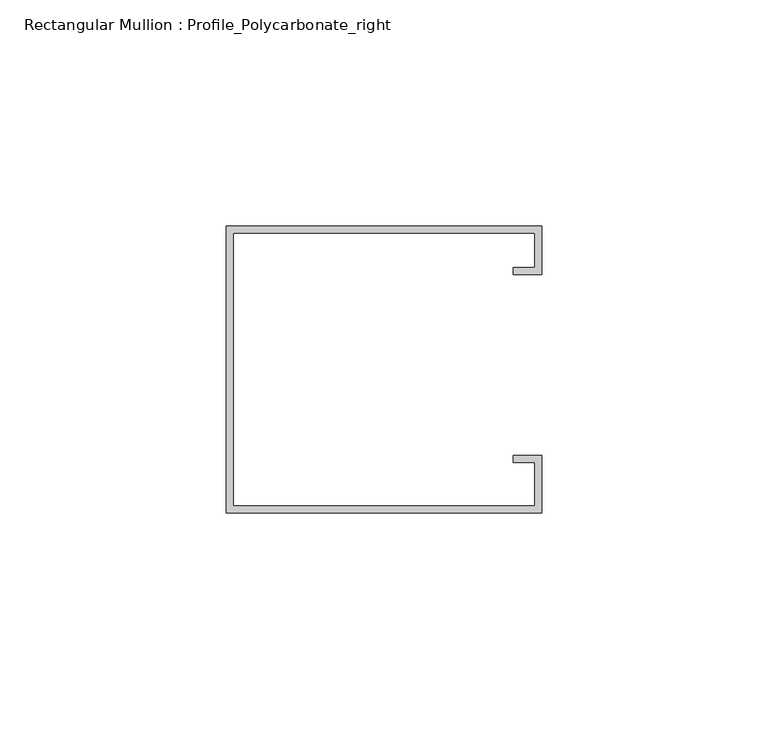
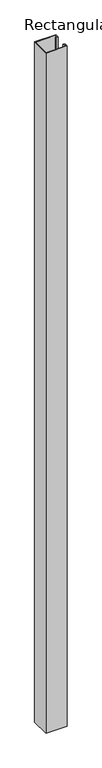
"""IFC4 building model written with IfcOpenShell, lengths in millimetres: member geometry, Rectangular Mullion : Profile_Polycarbonate_right."""

from ifc_helpers import new_model, si_unit, frame, origin, place, context, project, spatial, polyline, outline, extrude, source, transform, mapped, element, save


def rectangular_mullion_profile_polycarbonate_right_dcee4b73(model_context):
    return source(origin(), model_context, "Body", "SweptSolid", [
        extrude(outline(polyline([(0.0, -32.7), (0.0, 30.8), (69.85, 30.8), (69.85, 20.0), (63.5, 20.0), (63.5, 21.5875), (68.2625, 21.5875), (68.2625, 29.2125), (1.5875, 29.2125), (1.5875, -31.1125), (68.2625, -31.1125), (68.2625, -21.5875), (63.5, -21.5875), (63.5, -20.0), (69.85, -20.0), (69.85, -32.7), (0.0, -32.7)])), frame((0.0, 0.0, -2362.2), z_axis=(0.0, 0.0, 1.0), x_axis=(1.0, 0.0, 0.0)), (0.0, 0.0, 1.0), 2362.2),
    ])


if __name__ == "__main__":
    model = new_model("IFC4")
    model_context = context("Model", 3, world=origin())
    ifc_project = project(units=[si_unit("LENGTHUNIT", "METRE", prefix="MILLI")], contexts=[model_context])
    site = spatial("IfcSite", under=ifc_project)
    building = spatial("IfcBuilding", under=site)
    placement = place(None, origin())
    rectangular_mullion_profile_polycarbonate_right_shape = rectangular_mullion_profile_polycarbonate_right_dcee4b73(model_context)
    element("IfcMember", 1, ObjectType="Rectangular Mullion : Profile_Polycarbonate_right", at=placement, inside=building, context=model_context, shape_type="MappedRepresentation", body=[
        mapped(rectangular_mullion_profile_polycarbonate_right_shape, transform((0.0, 0.0, 0.0), x_axis=(1.0, 0.0, 0.0), y_axis=(0.0, 1.0, 0.0), z_axis=(0.0, 0.0, 1.0))),
    ])
    save(model, "model.ifc")

# Revit data of these elements
# Type "Rectangular Mullion : Profile_Polycarbonate_right"
#   built-in parameter 1007322 = 0.208333 (stored number, unit not read)
#   built-in parameter 1007321 = 0 (stored number, unit not read)
#   built-in parameter 1007320 = 0.00520833 (stored number, unit not read)
# Element 1 (IfcMember, "Rectangular Mullion : Profile_Polycarbonate_right")
#   Materials on its faces: "ALUMINUM PROFILE AT POLYCARBONATE PANEL"
# Materials
#   "ALUMINUM PROFILE AT POLYCARBONATE PANEL": class "Metal", colour RGB 244 244 244, transparency 0, Description = "Aluminum 6061", Cost = 0
